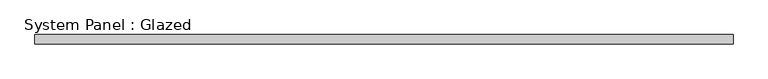
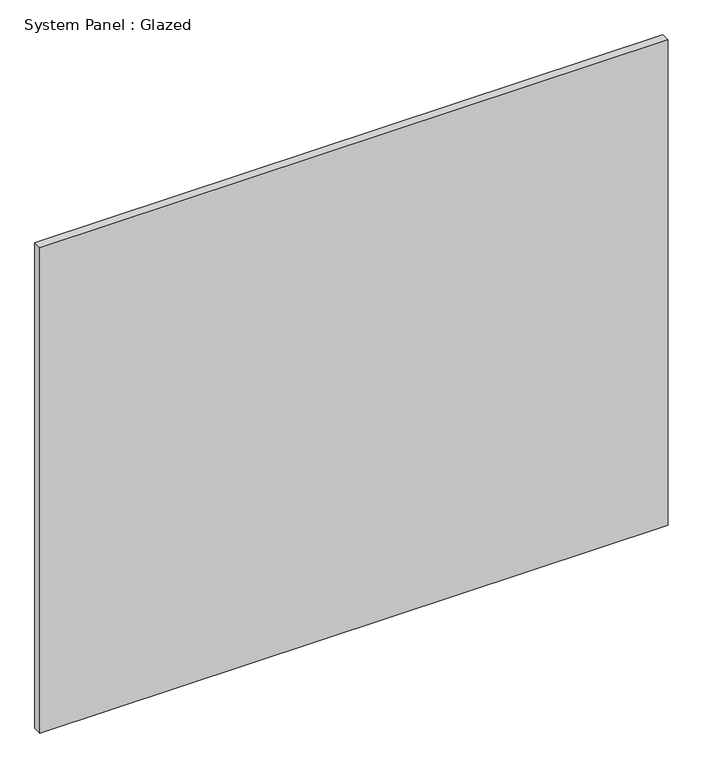
"""IFC4 building model written with IfcOpenShell, lengths in millimetres: plate geometry, System Panel : Glazed."""

from ifc_helpers import new_model, si_unit, origin, origin_with_axes, place, context, project, spatial, polyline, outline, extrude, source, transform, mapped, element, save


def system_panel_glazed_d72cc3ab(model_context):
    return source(origin(), model_context, "Body", "SweptSolid", [
        extrude(outline(polyline([(915.0000002, 24.5), (-915.0000002, 24.5), (-915.0000002, 49.5), (915.0000002, 49.5), (915.0000002, 24.5)])), origin_with_axes(), (0.0, 0.0, 1.0), 1494.0313026),
    ])


if __name__ == "__main__":
    model = new_model("IFC4")
    model_context = context("Model", 3, world=origin())
    ifc_project = project(units=[si_unit("LENGTHUNIT", "METRE", prefix="MILLI")], contexts=[model_context])
    site = spatial("IfcSite", under=ifc_project)
    building = spatial("IfcBuilding", under=site)
    placement = place(None, origin())
    system_panel_glazed_shape = system_panel_glazed_d72cc3ab(model_context)
    element("IfcPlate", 1, ObjectType="System Panel : Glazed", at=placement, inside=building, context=model_context, shape_type="MappedRepresentation", body=[
        mapped(system_panel_glazed_shape, transform((0.0, 0.0, 0.0), x_axis=(1.0, 0.0, 0.0), y_axis=(0.0, 1.0, 0.0), z_axis=(0.0, 0.0, 1.0))),
    ])
    save(model, "model.ifc")

# Revit data of these elements
# Element 1 (IfcPlate, "System Panel : Glazed")
#   Materials on its faces: "Glass"
# Materials
#   "Glass": class "Glass", colour RGB 218 227 224, transparency 0.85, Description = "Soda Lime Glass", Cost = 0
